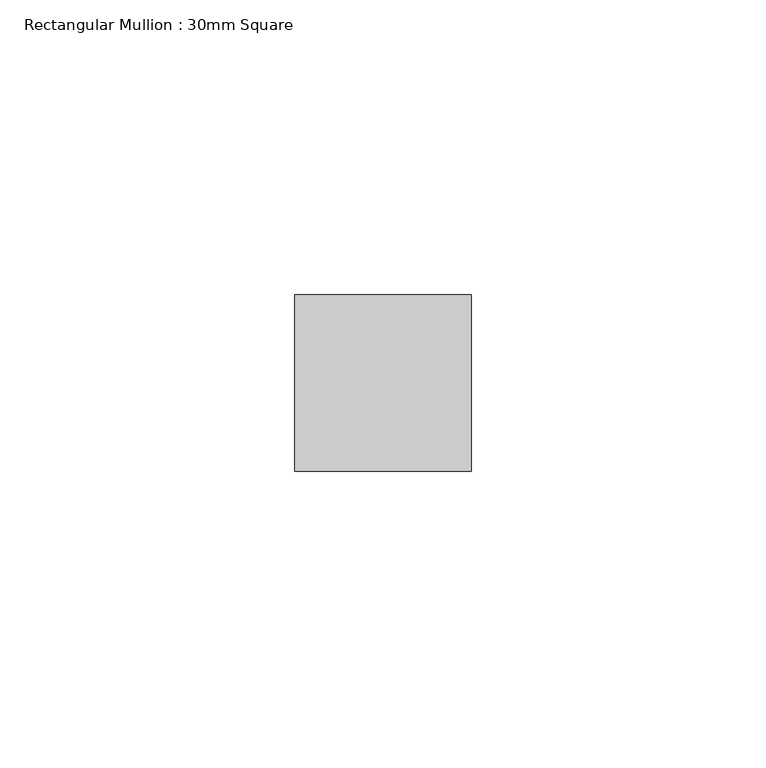
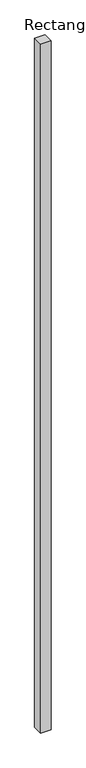
"""IFC4 building model written with IfcOpenShell, lengths in millimetres: member geometry, Rectangular Mullion : 30mm Square."""

from ifc_helpers import new_model, si_unit, frame, origin, place, context, project, spatial, polyline, outline, extrude, source, transform, mapped, element, save


def rectangular_mullion_30mm_square_c928f02b(model_context):
    return source(origin(), model_context, "Body", "SweptSolid", [
        extrude(outline(polyline([(15.0, 15.0), (15.0, -15.0), (-15.0, -15.0), (-15.0, 15.0), (15.0, 15.0)])), frame((0.0, 0.0, -2078.9136562), z_axis=(0.0, 0.0, 1.0), x_axis=(1.0, 0.0, 0.0)), (0.0, 0.0, 1.0), 2078.9136562),
    ])


if __name__ == "__main__":
    model = new_model("IFC4")
    model_context = context("Model", 3, world=origin())
    ifc_project = project(units=[si_unit("LENGTHUNIT", "METRE", prefix="MILLI")], contexts=[model_context])
    site = spatial("IfcSite", under=ifc_project)
    building = spatial("IfcBuilding", under=site)
    placement = place(None, origin())
    rectangular_mullion_30mm_square_shape = rectangular_mullion_30mm_square_c928f02b(model_context)
    element("IfcMember", 1, ObjectType="Rectangular Mullion : 30mm Square", at=placement, inside=building, context=model_context, shape_type="MappedRepresentation", body=[
        mapped(rectangular_mullion_30mm_square_shape, transform((0.0, 0.0, 0.0), x_axis=(1.0, 0.0, 0.0), y_axis=(0.0, 1.0, 0.0), z_axis=(0.0, 0.0, 1.0))),
    ])
    save(model, "model.ifc")

# Revit data of these elements
# Type "Rectangular Mullion : 30mm Square"
#   built-in parameter 1007304 = 0.0984252 (stored number, unit not read)
#   built-in parameter 1007301 = 0.0492126 (stored number, unit not read)
#   built-in parameter 1007300 = 0.0492126 (stored number, unit not read)
# Element 1 (IfcMember, "Rectangular Mullion : 30mm Square")
#   Materials on its faces: "Aluminum"
# Materials
#   "Aluminum": class "Metal", colour RGB 244 244 244, transparency 0, Description = "Aluminum 6061", Cost = 0
